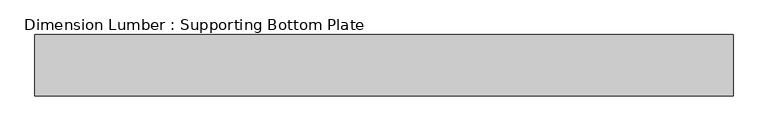
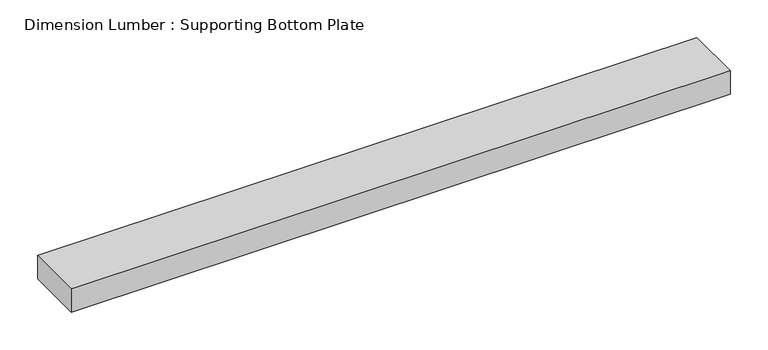
"""IFC4 building model written with IfcOpenShell, lengths in millimetres: beam geometry, Dimension Lumber : Supporting Bottom Plate."""

import ifcopenshell
import ifcopenshell.guid

model = None  # the IFC model being written
_history = None  # IfcOwnerHistory: only IFC2X3 demands one
_inside = {}  # id of a spatial element -> (the spatial element, [elements in it])
_under = {}  # id of a project, library or spatial element -> (it, [spatial elements below it])
_declared = {}  # id of a project -> (the project, [libraries it declares])
_typed = {}  # id of a type object -> (the type object, [elements of that type])
_made_of = {}  # id of a material, layer set ... -> (it, [elements and type objects made of it])


def new_model(schema):
    """Start an empty IFC model of exactly this schema.

    Asked for "IFC4X3", IfcOpenShell would pick the latest addendum, in which some entities
    have other attributes; the version numbers below select the first issue.
    IFC2X3 requires an IfcOwnerHistory on every rooted entity: one is made here for all.
    """
    global model, _history
    if schema == "IFC4X3":
        model = ifcopenshell.file(schema_version=(4, 3, 0, 0))
    else:
        model = ifcopenshell.file(schema=schema)
    _inside.clear()
    _under.clear()
    _declared.clear()
    _typed.clear()
    _made_of.clear()
    _history = None
    if model.schema == "IFC2X3":
        org = make("IfcOrganization", Name="unknown")
        user = make(
            "IfcPersonAndOrganization",
            ThePerson=make("IfcPerson", FamilyName="unknown"),
            TheOrganization=org,
        )
        app = make(
            "IfcApplication",
            ApplicationDeveloper=org,
            Version="unknown",
            ApplicationFullName="unknown",
            ApplicationIdentifier="unknown",
        )
        _history = make(
            "IfcOwnerHistory",
            OwningUser=user,
            OwningApplication=app,
            ChangeAction="ADDED",
            CreationDate=0,
        )
    return model


def make(cls, **values):
    """One entity of the class cls with the attributes given. An attribute that is None is left unset."""
    return model.create_entity(
        cls, **{name: value for name, value in values.items() if value is not None}
    )


def rooted(cls, **values):
    """An entity with a GlobalId (a new one), such as an element, a storey or a relation."""
    return make(cls, GlobalId=ifcopenshell.guid.new(), OwnerHistory=_history, **values)


def si_unit(unit_type, name, prefix=None):
    """IfcSIUnit, for example si_unit("LENGTHUNIT", "METRE", prefix="MILLI")."""
    return make("IfcSIUnit", UnitType=unit_type, Prefix=prefix, Name=name)


def assignment(units):
    """IfcUnitAssignment: the units of a project."""
    return None if units is None else make("IfcUnitAssignment", Units=units)


def point(xyz):
    """IfcCartesianPoint."""
    return None if xyz is None else make("IfcCartesianPoint", Coordinates=xyz)


def direction(xyz):
    """IfcDirection."""
    return None if xyz is None else make("IfcDirection", DirectionRatios=xyz)


def frame(location, z_axis=None, x_axis=None):
    """IfcAxis2Placement3D, a coordinate frame: its origin and axes. An axis left out is left unset."""
    return make(
        "IfcAxis2Placement3D",
        Location=point(location),
        Axis=direction(z_axis),
        RefDirection=direction(x_axis),
    )


def origin():
    """The frame at (0, 0, 0) with its axes left unset."""
    return frame((0.0, 0.0, 0.0))


def place(relative_to, where):
    """IfcLocalPlacement: puts the frame where relative to a parent placement (None: the world)."""
    return make(
        "IfcLocalPlacement", PlacementRelTo=relative_to, RelativePlacement=where
    )


def context(
    kind, dimensions, precision=None, world=None, true_north=None, identifier=None
):
    """IfcGeometricRepresentationContext, for example the 3D "Model" context."""
    return make(
        "IfcGeometricRepresentationContext",
        ContextIdentifier=identifier,
        ContextType=kind,
        CoordinateSpaceDimension=dimensions,
        Precision=precision,
        WorldCoordinateSystem=world,
        TrueNorth=true_north,
    )


def project(units=None, contexts=None):
    """IfcProject with its units and contexts."""
    return rooted(
        "IfcProject",
        Name="project",
        RepresentationContexts=contexts,
        UnitsInContext=assignment(units),
    )


def spatial(cls, under=None, at=None, **own):
    """A site, building, storey or space (cls), placed at a placement, below another one or the project."""
    s = rooted(cls, ObjectPlacement=at, **own)
    if under is not None:
        _under.setdefault(under.id(), (under, []))[1].append(s)
    return s


def polyline(points):
    """IfcPolyline through the points."""
    return make("IfcPolyline", Points=[point(p) for p in points])


def outline(outer, holes=None, kind="AREA"):
    """IfcArbitraryClosedProfileDef: a profile drawn as a closed curve; with holes, ...WithVoids."""
    if holes is None:
        return make("IfcArbitraryClosedProfileDef", ProfileType=kind, OuterCurve=outer)
    return make(
        "IfcArbitraryProfileDefWithVoids",
        ProfileType=kind,
        OuterCurve=outer,
        InnerCurves=holes,
    )


def extrude(swept, where, along, depth):
    """IfcExtrudedAreaSolid: the profile swept, set in the frame where, extruded along a direction by depth."""
    return make(
        "IfcExtrudedAreaSolid",
        SweptArea=swept,
        Position=where,
        ExtrudedDirection=direction(along),
        Depth=depth,
    )


def shape(context_of_items, identifier, shape_type, items):
    """IfcShapeRepresentation: the items that make up one representation, for example the "Body"."""
    return make(
        "IfcShapeRepresentation",
        ContextOfItems=context_of_items,
        RepresentationIdentifier=identifier,
        RepresentationType=shape_type,
        Items=items,
    )


def source(mapping_origin, context_of_items, identifier, shape_type, items):
    """IfcRepresentationMap: a shape defined once, which mapped items show again and again."""
    return make(
        "IfcRepresentationMap",
        MappingOrigin=mapping_origin,
        MappedRepresentation=shape(context_of_items, identifier, shape_type, items),
    )


def transform(
    local_origin,
    x_axis=None,
    y_axis=None,
    z_axis=None,
    scale=None,
    scale2=None,
    scale3=None,
    uniform=True,
):
    """IfcCartesianTransformationOperator3D, or its non-uniform kind. x_axis, y_axis, z_axis: its Axis1, 2, 3."""
    if uniform:
        return make(
            "IfcCartesianTransformationOperator3D",
            Axis1=direction(x_axis),
            Axis2=direction(y_axis),
            LocalOrigin=point(local_origin),
            Scale=scale,
            Axis3=direction(z_axis),
        )
    return make(
        "IfcCartesianTransformationOperator3DnonUniform",
        Axis1=direction(x_axis),
        Axis2=direction(y_axis),
        LocalOrigin=point(local_origin),
        Scale=scale,
        Axis3=direction(z_axis),
        Scale2=scale2,
        Scale3=scale3,
    )


def mapped(mapping_source, mapping_target):
    """IfcMappedItem: shows the shape of a source again, moved by a transform."""
    return make(
        "IfcMappedItem", MappingSource=mapping_source, MappingTarget=mapping_target
    )


def made_of(thing, what):
    """Note that an element or type object is made of a material, layer set ...; save() writes the relation."""
    if what is not None:
        _made_of.setdefault(what.id(), (what, []))[1].append(thing)
    return thing


def element(
    cls,
    number,
    at=None,
    inside=None,
    cuts=None,
    type_object=None,
    material=None,
    context=None,
    identifier="Body",
    shape_type=None,
    held_by="IfcProductDefinitionShape",
    body=None,
    shapes=None,
    **own,
):
    """One element of the class cls, such as IfcWall. Its Tag is "e" and its number.

    at: its placement. inside: the storey or other place that contains it. cuts: it is an
    opening in that element (IfcRelVoidsElement). A single representation is given by context,
    identifier, shape_type and body (its items); several are given by shapes. held_by: the class
    of the entity that holds the representations. save() writes the other relations.
    """
    e = rooted(cls, Tag="e%d" % number, ObjectPlacement=at, **own)
    if body is not None:
        shapes = [shape(context, identifier, shape_type, body)]
    if shapes is not None:
        e.Representation = make(held_by, Representations=shapes)
    if inside is not None:
        _inside.setdefault(inside.id(), (inside, []))[1].append(e)
    if cuts is not None:
        rooted(
            "IfcRelVoidsElement", RelatingBuildingElement=cuts, RelatedOpeningElement=e
        )
    if type_object is not None:
        _typed.setdefault(type_object.id(), (type_object, []))[1].append(e)
    return made_of(e, material)


def aggregate(whole, parts):
    """IfcRelAggregates: a whole, such as a stair, and the parts it consists of."""
    return rooted("IfcRelAggregates", RelatingObject=whole, RelatedObjects=parts)


def save(model, path):
    """Write the relations noted so far, then the file.

    IfcRelAggregates (storeys below a building ...), IfcRelContainedInSpatialStructure (elements
    in a storey), IfcRelDefinesByType, IfcRelAssociatesMaterial and IfcRelDeclares: one each for
    every whole, place, type object, material and project.
    """
    for whole, parts in _under.values():
        aggregate(whole, parts)
    for where, things in _inside.values():
        rooted(
            "IfcRelContainedInSpatialStructure",
            RelatedElements=things,
            RelatingStructure=where,
        )
    for kind, things in _typed.values():
        rooted("IfcRelDefinesByType", RelatedObjects=things, RelatingType=kind)
    for what, things in _made_of.values():
        rooted("IfcRelAssociatesMaterial", RelatedObjects=things, RelatingMaterial=what)
    for by, libraries in _declared.values():
        rooted("IfcRelDeclares", RelatingContext=by, RelatedDefinitions=libraries)
    model.write(path)


def dimension_lumber_supporting_bottom_plate_c78b9630(model_context):
    return source(origin(), model_context, "Body", "SweptSolid", [
        extrude(outline(polyline([(488.95, 44.45), (488.95, -44.45), (-521.890625, -44.45), (-521.890625, 44.45), (488.95, 44.45)])), frame((0.0, 0.0, -19.05), z_axis=(0.0, 0.0, 1.0), x_axis=(1.0, 0.0, 0.0)), (0.0, 0.0, 1.0), 38.1),
    ])


if __name__ == "__main__":
    model = new_model("IFC4")
    model_context = context("Model", 3, world=origin())
    ifc_project = project(units=[si_unit("LENGTHUNIT", "METRE", prefix="MILLI")], contexts=[model_context])
    site = spatial("IfcSite", under=ifc_project)
    building = spatial("IfcBuilding", under=site)
    placement = place(None, origin())
    dimension_lumber_supporting_bottom_plate_shape = dimension_lumber_supporting_bottom_plate_c78b9630(model_context)
    element("IfcBeam", 1, ObjectType="Dimension Lumber : Supporting Bottom Plate", at=placement, inside=building, context=model_context, shape_type="MappedRepresentation", body=[
        mapped(dimension_lumber_supporting_bottom_plate_shape, transform((0.0, 0.0, 0.0), x_axis=(1.0, 0.0, 0.0), y_axis=(0.0, 1.0, 0.0), z_axis=(0.0, 0.0, 1.0))),
    ])
    save(model, "model.ifc")

# Revit data of these elements
# Type "Dimension Lumber : Supporting Bottom Plate"
#   Assembly Code = "B10"
#   A = 0.0364583 SF
#   Length [instance default] = 5' - 0"
#   b = 0' - 3 1/2"
#   d = 0' - 1 1/2"
#   Structural Material [instance default] = Softwood, Lumber
# Element 1 (IfcBeam, "Dimension Lumber : Supporting Bottom Plate")
#   Structural Material = Douglas Fir #2
#   Materials on its faces: "Douglas Fir #2"
# Materials
#   "Softwood, Lumber": class "Wood", colour RGB 223 192 134, transparency 0, Description = "Pinus Echinata", Cost = 0
#   "Douglas Fir #2": class "Wood", colour RGB 223 192 134, transparency 0, Description = "Pinus Echinata", Cost = 0
